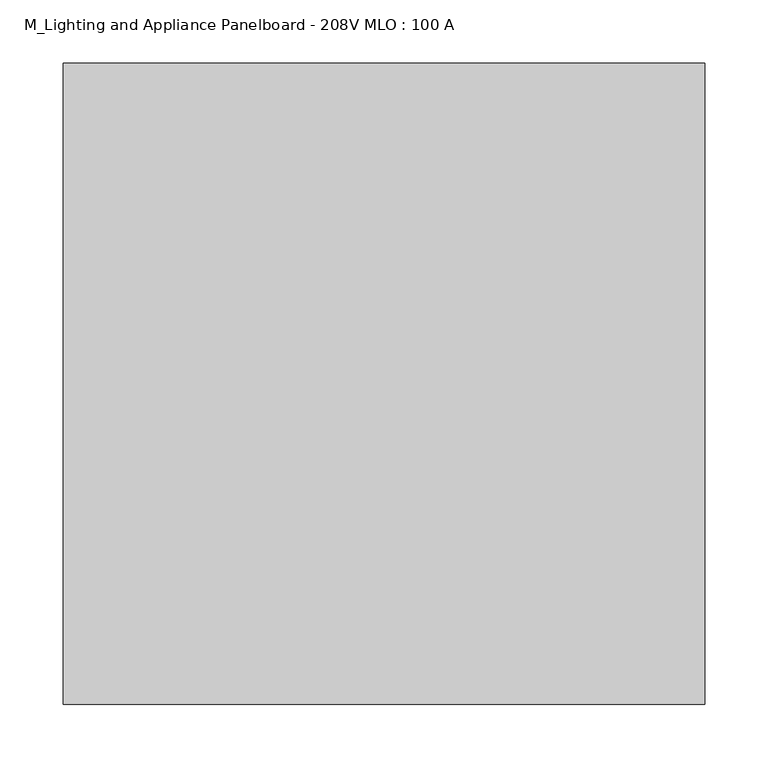
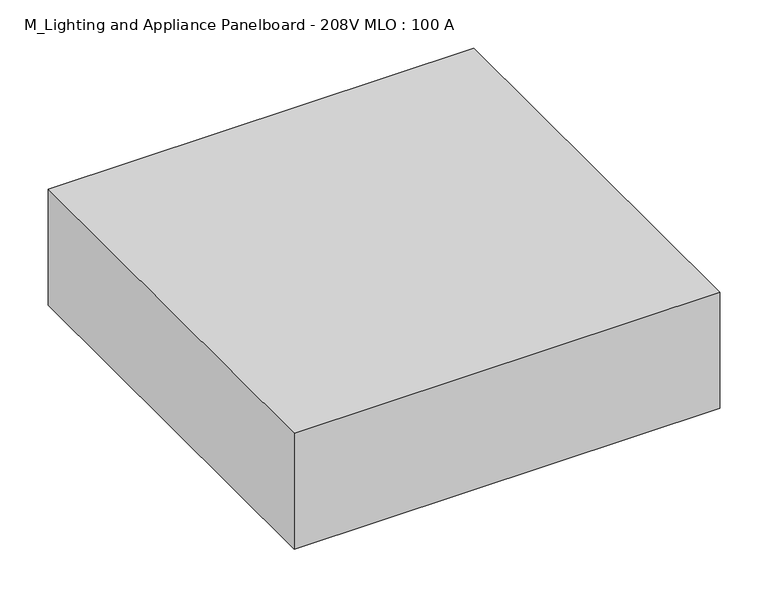
"""IFC4 building model written with IfcOpenShell, lengths in millimetres: proxy geometry, M_Lighting and Appliance Panelboard - 208V MLO : 100 A."""

import ifcopenshell
import ifcopenshell.guid

model = None  # the IFC model being written
_history = None  # IfcOwnerHistory: only IFC2X3 demands one
_inside = {}  # id of a spatial element -> (the spatial element, [elements in it])
_under = {}  # id of a project, library or spatial element -> (it, [spatial elements below it])
_declared = {}  # id of a project -> (the project, [libraries it declares])
_typed = {}  # id of a type object -> (the type object, [elements of that type])
_made_of = {}  # id of a material, layer set ... -> (it, [elements and type objects made of it])


def new_model(schema):
    """Start an empty IFC model of exactly this schema.

    Asked for "IFC4X3", IfcOpenShell would pick the latest addendum, in which some entities
    have other attributes; the version numbers below select the first issue.
    IFC2X3 requires an IfcOwnerHistory on every rooted entity: one is made here for all.
    """
    global model, _history
    if schema == "IFC4X3":
        model = ifcopenshell.file(schema_version=(4, 3, 0, 0))
    else:
        model = ifcopenshell.file(schema=schema)
    _inside.clear()
    _under.clear()
    _declared.clear()
    _typed.clear()
    _made_of.clear()
    _history = None
    if model.schema == "IFC2X3":
        org = make("IfcOrganization", Name="unknown")
        user = make(
            "IfcPersonAndOrganization",
            ThePerson=make("IfcPerson", FamilyName="unknown"),
            TheOrganization=org,
        )
        app = make(
            "IfcApplication",
            ApplicationDeveloper=org,
            Version="unknown",
            ApplicationFullName="unknown",
            ApplicationIdentifier="unknown",
        )
        _history = make(
            "IfcOwnerHistory",
            OwningUser=user,
            OwningApplication=app,
            ChangeAction="ADDED",
            CreationDate=0,
        )
    return model


def make(cls, **values):
    """One entity of the class cls with the attributes given. An attribute that is None is left unset."""
    return model.create_entity(
        cls, **{name: value for name, value in values.items() if value is not None}
    )


def rooted(cls, **values):
    """An entity with a GlobalId (a new one), such as an element, a storey or a relation."""
    return make(cls, GlobalId=ifcopenshell.guid.new(), OwnerHistory=_history, **values)


def si_unit(unit_type, name, prefix=None):
    """IfcSIUnit, for example si_unit("LENGTHUNIT", "METRE", prefix="MILLI")."""
    return make("IfcSIUnit", UnitType=unit_type, Prefix=prefix, Name=name)


def assignment(units):
    """IfcUnitAssignment: the units of a project."""
    return None if units is None else make("IfcUnitAssignment", Units=units)


def point(xyz):
    """IfcCartesianPoint."""
    return None if xyz is None else make("IfcCartesianPoint", Coordinates=xyz)


def direction(xyz):
    """IfcDirection."""
    return None if xyz is None else make("IfcDirection", DirectionRatios=xyz)


def frame(location, z_axis=None, x_axis=None):
    """IfcAxis2Placement3D, a coordinate frame: its origin and axes. An axis left out is left unset."""
    return make(
        "IfcAxis2Placement3D",
        Location=point(location),
        Axis=direction(z_axis),
        RefDirection=direction(x_axis),
    )


def origin():
    """The frame at (0, 0, 0) with its axes left unset."""
    return frame((0.0, 0.0, 0.0))


def place(relative_to, where):
    """IfcLocalPlacement: puts the frame where relative to a parent placement (None: the world)."""
    return make(
        "IfcLocalPlacement", PlacementRelTo=relative_to, RelativePlacement=where
    )


def context(
    kind, dimensions, precision=None, world=None, true_north=None, identifier=None
):
    """IfcGeometricRepresentationContext, for example the 3D "Model" context."""
    return make(
        "IfcGeometricRepresentationContext",
        ContextIdentifier=identifier,
        ContextType=kind,
        CoordinateSpaceDimension=dimensions,
        Precision=precision,
        WorldCoordinateSystem=world,
        TrueNorth=true_north,
    )


def project(units=None, contexts=None):
    """IfcProject with its units and contexts."""
    return rooted(
        "IfcProject",
        Name="project",
        RepresentationContexts=contexts,
        UnitsInContext=assignment(units),
    )


def spatial(cls, under=None, at=None, **own):
    """A site, building, storey or space (cls), placed at a placement, below another one or the project."""
    s = rooted(cls, ObjectPlacement=at, **own)
    if under is not None:
        _under.setdefault(under.id(), (under, []))[1].append(s)
    return s


def polyline(points):
    """IfcPolyline through the points."""
    return make("IfcPolyline", Points=[point(p) for p in points])


def outline(outer, holes=None, kind="AREA"):
    """IfcArbitraryClosedProfileDef: a profile drawn as a closed curve; with holes, ...WithVoids."""
    if holes is None:
        return make("IfcArbitraryClosedProfileDef", ProfileType=kind, OuterCurve=outer)
    return make(
        "IfcArbitraryProfileDefWithVoids",
        ProfileType=kind,
        OuterCurve=outer,
        InnerCurves=holes,
    )


def extrude(swept, where, along, depth):
    """IfcExtrudedAreaSolid: the profile swept, set in the frame where, extruded along a direction by depth."""
    return make(
        "IfcExtrudedAreaSolid",
        SweptArea=swept,
        Position=where,
        ExtrudedDirection=direction(along),
        Depth=depth,
    )


def shape(context_of_items, identifier, shape_type, items):
    """IfcShapeRepresentation: the items that make up one representation, for example the "Body"."""
    return make(
        "IfcShapeRepresentation",
        ContextOfItems=context_of_items,
        RepresentationIdentifier=identifier,
        RepresentationType=shape_type,
        Items=items,
    )


def source(mapping_origin, context_of_items, identifier, shape_type, items):
    """IfcRepresentationMap: a shape defined once, which mapped items show again and again."""
    return make(
        "IfcRepresentationMap",
        MappingOrigin=mapping_origin,
        MappedRepresentation=shape(context_of_items, identifier, shape_type, items),
    )


def transform(
    local_origin,
    x_axis=None,
    y_axis=None,
    z_axis=None,
    scale=None,
    scale2=None,
    scale3=None,
    uniform=True,
):
    """IfcCartesianTransformationOperator3D, or its non-uniform kind. x_axis, y_axis, z_axis: its Axis1, 2, 3."""
    if uniform:
        return make(
            "IfcCartesianTransformationOperator3D",
            Axis1=direction(x_axis),
            Axis2=direction(y_axis),
            LocalOrigin=point(local_origin),
            Scale=scale,
            Axis3=direction(z_axis),
        )
    return make(
        "IfcCartesianTransformationOperator3DnonUniform",
        Axis1=direction(x_axis),
        Axis2=direction(y_axis),
        LocalOrigin=point(local_origin),
        Scale=scale,
        Axis3=direction(z_axis),
        Scale2=scale2,
        Scale3=scale3,
    )


def mapped(mapping_source, mapping_target):
    """IfcMappedItem: shows the shape of a source again, moved by a transform."""
    return make(
        "IfcMappedItem", MappingSource=mapping_source, MappingTarget=mapping_target
    )


def made_of(thing, what):
    """Note that an element or type object is made of a material, layer set ...; save() writes the relation."""
    if what is not None:
        _made_of.setdefault(what.id(), (what, []))[1].append(thing)
    return thing


def element(
    cls,
    number,
    at=None,
    inside=None,
    cuts=None,
    type_object=None,
    material=None,
    context=None,
    identifier="Body",
    shape_type=None,
    held_by="IfcProductDefinitionShape",
    body=None,
    shapes=None,
    **own,
):
    """One element of the class cls, such as IfcWall. Its Tag is "e" and its number.

    at: its placement. inside: the storey or other place that contains it. cuts: it is an
    opening in that element (IfcRelVoidsElement). A single representation is given by context,
    identifier, shape_type and body (its items); several are given by shapes. held_by: the class
    of the entity that holds the representations. save() writes the other relations.
    """
    e = rooted(cls, Tag="e%d" % number, ObjectPlacement=at, **own)
    if body is not None:
        shapes = [shape(context, identifier, shape_type, body)]
    if shapes is not None:
        e.Representation = make(held_by, Representations=shapes)
    if inside is not None:
        _inside.setdefault(inside.id(), (inside, []))[1].append(e)
    if cuts is not None:
        rooted(
            "IfcRelVoidsElement", RelatingBuildingElement=cuts, RelatedOpeningElement=e
        )
    if type_object is not None:
        _typed.setdefault(type_object.id(), (type_object, []))[1].append(e)
    return made_of(e, material)


def aggregate(whole, parts):
    """IfcRelAggregates: a whole, such as a stair, and the parts it consists of."""
    return rooted("IfcRelAggregates", RelatingObject=whole, RelatedObjects=parts)


def save(model, path):
    """Write the relations noted so far, then the file.

    IfcRelAggregates (storeys below a building ...), IfcRelContainedInSpatialStructure (elements
    in a storey), IfcRelDefinesByType, IfcRelAssociatesMaterial and IfcRelDeclares: one each for
    every whole, place, type object, material and project.
    """
    for whole, parts in _under.values():
        aggregate(whole, parts)
    for where, things in _inside.values():
        rooted(
            "IfcRelContainedInSpatialStructure",
            RelatedElements=things,
            RelatingStructure=where,
        )
    for kind, things in _typed.values():
        rooted("IfcRelDefinesByType", RelatedObjects=things, RelatingType=kind)
    for what, things in _made_of.values():
        rooted("IfcRelAssociatesMaterial", RelatedObjects=things, RelatingMaterial=what)
    for by, libraries in _declared.values():
        rooted("IfcRelDeclares", RelatingContext=by, RelatedDefinitions=libraries)
    model.write(path)


def m_lighting_and_appliance_panelboard_208v_mlo_100_a_deb79597(model_context):
    return source(origin(), model_context, "Body", "SweptSolid", [
        extrude(outline(polyline([(254.0, -165.1), (254.0, -673.1), (-254.0, -673.1), (-254.0, -165.1), (254.0, -165.1)])), frame((0.0, 0.0, -146.1), z_axis=(0.0, 0.0, 1.0), x_axis=(1.0, 0.0, 0.0)), (0.0, 0.0, 1.0), 146.1),
    ])


if __name__ == "__main__":
    model = new_model("IFC4")
    model_context = context("Model", 3, world=origin())
    ifc_project = project(units=[si_unit("LENGTHUNIT", "METRE", prefix="MILLI")], contexts=[model_context])
    site = spatial("IfcSite", under=ifc_project)
    building = spatial("IfcBuilding", under=site)
    placement = place(None, origin())
    m_lighting_and_appliance_panelboard_208v_mlo_100_a_shape = m_lighting_and_appliance_panelboard_208v_mlo_100_a_deb79597(model_context)
    element("IfcBuildingElementProxy", 1, Name="M_Lighting and Appliance Panelboard - 208V MLO : 100 A", ObjectType="M_Lighting and Appliance Panelboard - 208V MLO : 100 A", at=placement, inside=building, context=model_context, shape_type="MappedRepresentation", body=[
        mapped(m_lighting_and_appliance_panelboard_208v_mlo_100_a_shape, transform((0.0, 0.0, 0.0), x_axis=(1.0, 0.0, 0.0), y_axis=(0.0, 1.0, 0.0), z_axis=(0.0, 0.0, 1.0))),
    ])
    save(model, "model.ifc")

# Revit data of these elements
# Type "M_Lighting and Appliance Panelboard - 208V MLO : 100 A"
#   built-in parameter 1140081 [instance default] = "Recessed"
#   built-in parameter 1140083 [instance default] = "Type 1"
#   Width = 508 mm
#   built-in parameter 1140082 [instance default] = 100 (stored number, unit not read)
#   Height [instance default] = 508 mm
#   Depth = 146.1 mm
#   Default Elevation = 1200 mm
#   42 Circuit Height = 1041.4 mm
#   30 Circuit Height = 660.4 mm
#   24 Circuit Height = 584.2 mm
#   12 Circuit Height = 508 mm
#   built-in parameter 1140079 [instance default] = 12
#   Load Classification = Other
